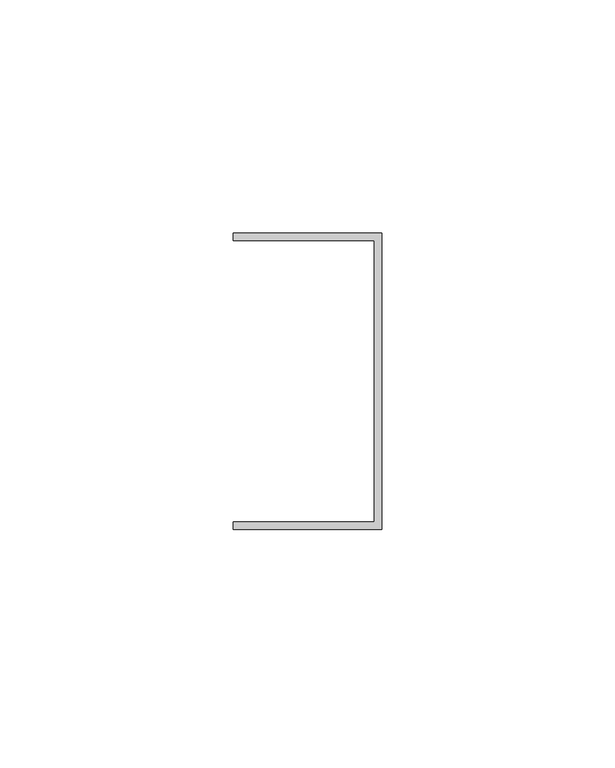
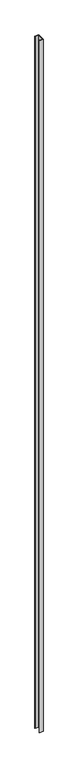
"""IFC4 building model written with IfcOpenShell, lengths in millimetres: proxy geometry, Generic Models 7:Generic Models 1:3:Generic Models 1:3 : Generic Models 7:Generic Models 1:305549:3:Generic Models 1:3:Generic Models 1:3 : Generic Models 7:Generic Models 1:305549:3 : Generic Models 7:Generic Models 1:3:Generic Models 1:3 : Generic Models 7:Generic Models 1:305549:301244:39 : Generic Models 7:Generic Models 1:3:Generic Models 1:3 : Generic Models 7:Generic Models 1:305549:3:Generic Models 1:3:Generic Models 1:3 : Generic Models 7:Generic Models 1:305549:3 : Generic Models 7:Generic Models 1:3:Generic Models 1:3 : Generic Models 7:Generic Models 1:305549:301244:308848."""

from ifc_helpers import new_model, si_unit, origin, origin_with_axes, place, context, project, spatial, polyline, outline, extrude, source, transform, mapped, element, save


def generic_models_3fde2765(model_context):
    return source(origin(), model_context, "Body", "SweptSolid", [
        extrude(outline(polyline([(803158.9132437, -579013.3913841), (803158.9132437, -579076.8913841), (803127.1632437, -579076.8913841), (803127.1632437, -579075.3038841), (803157.3257437, -579075.3038841), (803157.3257437, -579014.9788841), (803127.1632437, -579014.9788841), (803127.1632437, -579013.3913841), (803158.9132437, -579013.3913841)])), origin_with_axes(), (0.0, 0.0, 1.0), 6134.1),
    ])


if __name__ == "__main__":
    model = new_model("IFC4")
    model_context = context("Model", 3, world=origin())
    ifc_project = project(units=[si_unit("LENGTHUNIT", "METRE", prefix="MILLI")], contexts=[model_context])
    site = spatial("IfcSite", under=ifc_project)
    building = spatial("IfcBuilding", under=site)
    placement = place(None, origin())
    generic_models_shape = generic_models_3fde2765(model_context)
    element("IfcBuildingElementProxy", 1, Name="Generic Models 7:Generic Models 1:3:Generic Models 1:3 : Generic Models 7:Generic Models 1:305549:3:Generic Models 1:3:Generic Models 1:3 : Generic Models 7:Generic Models 1:305549:3 : Generic Models 7:Generic Models 1:3:Generic Models 1:3 : Generic Models 7:Generic Models 1:305549:301244:39 : Generic Models 7:Generic Models 1:3:Generic Models 1:3 : Generic Models 7:Generic Models 1:305549:3:Generic Models 1:3:Generic Models 1:3 : Generic Models 7:Generic Models 1:305549:3 : Generic Models 7:Generic Models 1:3:Generic Models 1:3 : Generic Models 7:Generic Models 1:305549:301244:308848", ObjectType="Generic Models 7:Generic Models 1:3:Generic Models 1:3 : Generic Models 7:Generic Models 1:305549:3:Generic Models 1:3:Generic Models 1:3 : Generic Models 7:Generic Models 1:305549:3 : Generic Models 7:Generic Models 1:3:Generic Models 1:3 : Generic Models 7:Generic Models 1:305549:301244:39 : Generic Models 7:Generic Models 1:3:Generic Models 1:3 : Generic Models 7:Generic Models 1:305549:3:Generic Models 1:3:Generic Models 1:3 : Generic Models 7:Generic Models 1:305549:3 : Generic Models 7:Generic Models 1:3:Generic Models 1:3 : Generic Models 7:Generic Models 1:305549:301244:308848", at=placement, inside=building, context=model_context, shape_type="MappedRepresentation", body=[
        mapped(generic_models_shape, transform((0.0, 0.0, 0.0), x_axis=(1.0, 0.0, 0.0), y_axis=(0.0, 1.0, 0.0), z_axis=(0.0, 0.0, 1.0))),
    ])
    save(model, "model.ifc")

# Revit data of these elements
# Type "Generic Models 7:Generic Models 1:3:Generic Models 1:3 : Generic Models 7:Generic Models 1:305549:3:Generic Models 1:3:Generic Models 1:3 : Generic Models 7:Generic Models 1:305549:3 : Generic Models 7:Generic Models 1:3:Generic Models 1:3 : Generic Models 7:Generic Models 1:305549:301244:39 : Generic Models 7:Generic Models 1:3:Generic Models 1:3 : Generic Models 7:Generic Models 1:305549:3:Generic Models 1:3:Generic Models 1:3 : Generic Models 7:Generic Models 1:305549:3 : Generic Models 7:Generic Models 1:3:Generic Models 1:3 : Generic Models 7:Generic Models 1:305549:301244:308848"
#   NameOverride = "Generic Models 7:Generic Models 1:3:Generic Models 1:3 : Generic Models 7:Generic Models 1:305549:3:Generic Models 1:3:Generic Models 1:3 : Generic Models 7:Generic Models 1:305549:3 : Generic Models 7:Generic Models 1:3:Generic Models 1:3 : Generic Models 7:Generic Models 1:305549:301244:308848"
#   ObjectTypeOverride = "Generic Models 1:3:Generic Models 1:3 : Generic Models 7:Generic Models 1:305549:3 : Generic Models 7:Generic Models 1:3:Generic Models 1:3 : Generic Models 7:Generic Models 1:305549:301244"
#   Reference = "Generic Models 1"
#   Tag = "308848"
# Element 1 (IfcBuildingElementProxy, "Generic Models 7:Generic Models 1:3:Generic Models 1:3 : Generic Models 7:Generic Models 1:305549:3:Generic Models 1:3:Generic Models 1:3 : Generic Models 7:Generic Models 1:305549:3 : Generic Models 7:Generic Models 1:3:Generic Models 1:3 : Generic Models 7:Generic Models 1:305549:301244:39 : Generic Models 7:Generic Models 1:3:Generic Models 1:3 : Generic Models 7:Generic Models 1:305549:3:Generic Models 1:3:Generic Models 1:3 : Generic Models 7:Generic Models 1:305549:3 : Generic Models 7:Generic Models 1:3:Generic Models 1:3 : Generic Models 7:Generic Models 1:305549:301244:308848")
#   Materials on its faces: "GALVANIZED U-CHANNEL (250T125-33)"
# Materials
#   "GALVANIZED U-CHANNEL (250T125-33)": class "Unassigned", colour RGB 202 201 200, transparency 0, Keynote = "M05451300.02", Cost = 0
